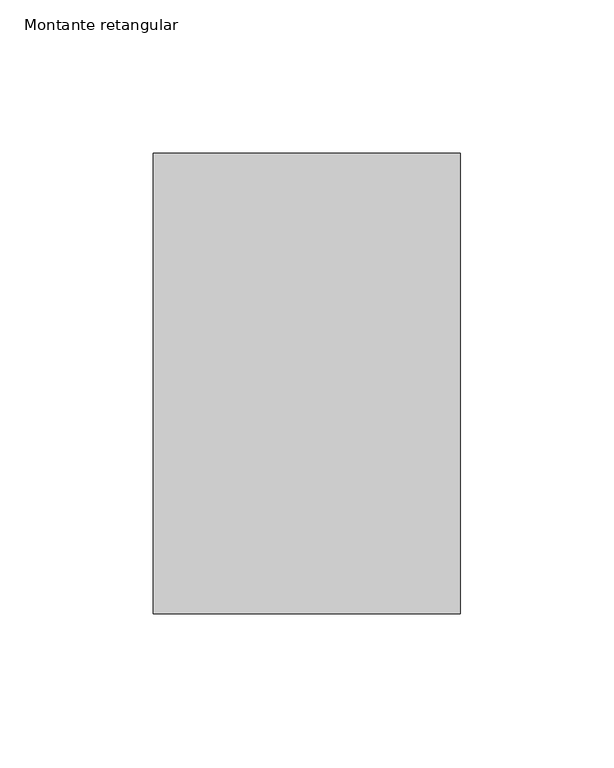
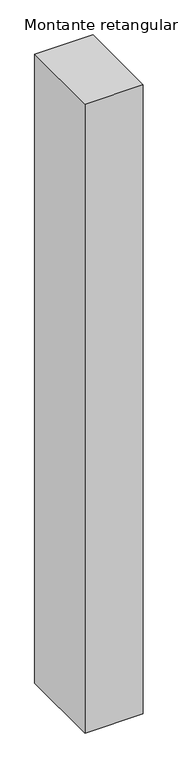
"""IFC4 building model written with IfcOpenShell, lengths in millimetres: member geometry, Montante retangular : CC_100 X 150  mm."""

import ifcopenshell
import ifcopenshell.guid

model = None  # the IFC model being written
_history = None  # IfcOwnerHistory: only IFC2X3 demands one
_inside = {}  # id of a spatial element -> (the spatial element, [elements in it])
_under = {}  # id of a project, library or spatial element -> (it, [spatial elements below it])
_declared = {}  # id of a project -> (the project, [libraries it declares])
_typed = {}  # id of a type object -> (the type object, [elements of that type])
_made_of = {}  # id of a material, layer set ... -> (it, [elements and type objects made of it])


def new_model(schema):
    """Start an empty IFC model of exactly this schema.

    Asked for "IFC4X3", IfcOpenShell would pick the latest addendum, in which some entities
    have other attributes; the version numbers below select the first issue.
    IFC2X3 requires an IfcOwnerHistory on every rooted entity: one is made here for all.
    """
    global model, _history
    if schema == "IFC4X3":
        model = ifcopenshell.file(schema_version=(4, 3, 0, 0))
    else:
        model = ifcopenshell.file(schema=schema)
    _inside.clear()
    _under.clear()
    _declared.clear()
    _typed.clear()
    _made_of.clear()
    _history = None
    if model.schema == "IFC2X3":
        org = make("IfcOrganization", Name="unknown")
        user = make(
            "IfcPersonAndOrganization",
            ThePerson=make("IfcPerson", FamilyName="unknown"),
            TheOrganization=org,
        )
        app = make(
            "IfcApplication",
            ApplicationDeveloper=org,
            Version="unknown",
            ApplicationFullName="unknown",
            ApplicationIdentifier="unknown",
        )
        _history = make(
            "IfcOwnerHistory",
            OwningUser=user,
            OwningApplication=app,
            ChangeAction="ADDED",
            CreationDate=0,
        )
    return model


def make(cls, **values):
    """One entity of the class cls with the attributes given. An attribute that is None is left unset."""
    return model.create_entity(
        cls, **{name: value for name, value in values.items() if value is not None}
    )


def rooted(cls, **values):
    """An entity with a GlobalId (a new one), such as an element, a storey or a relation."""
    return make(cls, GlobalId=ifcopenshell.guid.new(), OwnerHistory=_history, **values)


def si_unit(unit_type, name, prefix=None):
    """IfcSIUnit, for example si_unit("LENGTHUNIT", "METRE", prefix="MILLI")."""
    return make("IfcSIUnit", UnitType=unit_type, Prefix=prefix, Name=name)


def assignment(units):
    """IfcUnitAssignment: the units of a project."""
    return None if units is None else make("IfcUnitAssignment", Units=units)


def point(xyz):
    """IfcCartesianPoint."""
    return None if xyz is None else make("IfcCartesianPoint", Coordinates=xyz)


def direction(xyz):
    """IfcDirection."""
    return None if xyz is None else make("IfcDirection", DirectionRatios=xyz)


def frame(location, z_axis=None, x_axis=None):
    """IfcAxis2Placement3D, a coordinate frame: its origin and axes. An axis left out is left unset."""
    return make(
        "IfcAxis2Placement3D",
        Location=point(location),
        Axis=direction(z_axis),
        RefDirection=direction(x_axis),
    )


def origin():
    """The frame at (0, 0, 0) with its axes left unset."""
    return frame((0.0, 0.0, 0.0))


def place(relative_to, where):
    """IfcLocalPlacement: puts the frame where relative to a parent placement (None: the world)."""
    return make(
        "IfcLocalPlacement", PlacementRelTo=relative_to, RelativePlacement=where
    )


def context(
    kind, dimensions, precision=None, world=None, true_north=None, identifier=None
):
    """IfcGeometricRepresentationContext, for example the 3D "Model" context."""
    return make(
        "IfcGeometricRepresentationContext",
        ContextIdentifier=identifier,
        ContextType=kind,
        CoordinateSpaceDimension=dimensions,
        Precision=precision,
        WorldCoordinateSystem=world,
        TrueNorth=true_north,
    )


def project(units=None, contexts=None):
    """IfcProject with its units and contexts."""
    return rooted(
        "IfcProject",
        Name="project",
        RepresentationContexts=contexts,
        UnitsInContext=assignment(units),
    )


def spatial(cls, under=None, at=None, **own):
    """A site, building, storey or space (cls), placed at a placement, below another one or the project."""
    s = rooted(cls, ObjectPlacement=at, **own)
    if under is not None:
        _under.setdefault(under.id(), (under, []))[1].append(s)
    return s


def polyline(points):
    """IfcPolyline through the points."""
    return make("IfcPolyline", Points=[point(p) for p in points])


def outline(outer, holes=None, kind="AREA"):
    """IfcArbitraryClosedProfileDef: a profile drawn as a closed curve; with holes, ...WithVoids."""
    if holes is None:
        return make("IfcArbitraryClosedProfileDef", ProfileType=kind, OuterCurve=outer)
    return make(
        "IfcArbitraryProfileDefWithVoids",
        ProfileType=kind,
        OuterCurve=outer,
        InnerCurves=holes,
    )


def extrude(swept, where, along, depth):
    """IfcExtrudedAreaSolid: the profile swept, set in the frame where, extruded along a direction by depth."""
    return make(
        "IfcExtrudedAreaSolid",
        SweptArea=swept,
        Position=where,
        ExtrudedDirection=direction(along),
        Depth=depth,
    )


def shape(context_of_items, identifier, shape_type, items):
    """IfcShapeRepresentation: the items that make up one representation, for example the "Body"."""
    return make(
        "IfcShapeRepresentation",
        ContextOfItems=context_of_items,
        RepresentationIdentifier=identifier,
        RepresentationType=shape_type,
        Items=items,
    )


def source(mapping_origin, context_of_items, identifier, shape_type, items):
    """IfcRepresentationMap: a shape defined once, which mapped items show again and again."""
    return make(
        "IfcRepresentationMap",
        MappingOrigin=mapping_origin,
        MappedRepresentation=shape(context_of_items, identifier, shape_type, items),
    )


def transform(
    local_origin,
    x_axis=None,
    y_axis=None,
    z_axis=None,
    scale=None,
    scale2=None,
    scale3=None,
    uniform=True,
):
    """IfcCartesianTransformationOperator3D, or its non-uniform kind. x_axis, y_axis, z_axis: its Axis1, 2, 3."""
    if uniform:
        return make(
            "IfcCartesianTransformationOperator3D",
            Axis1=direction(x_axis),
            Axis2=direction(y_axis),
            LocalOrigin=point(local_origin),
            Scale=scale,
            Axis3=direction(z_axis),
        )
    return make(
        "IfcCartesianTransformationOperator3DnonUniform",
        Axis1=direction(x_axis),
        Axis2=direction(y_axis),
        LocalOrigin=point(local_origin),
        Scale=scale,
        Axis3=direction(z_axis),
        Scale2=scale2,
        Scale3=scale3,
    )


def mapped(mapping_source, mapping_target):
    """IfcMappedItem: shows the shape of a source again, moved by a transform."""
    return make(
        "IfcMappedItem", MappingSource=mapping_source, MappingTarget=mapping_target
    )


def made_of(thing, what):
    """Note that an element or type object is made of a material, layer set ...; save() writes the relation."""
    if what is not None:
        _made_of.setdefault(what.id(), (what, []))[1].append(thing)
    return thing


def element(
    cls,
    number,
    at=None,
    inside=None,
    cuts=None,
    type_object=None,
    material=None,
    context=None,
    identifier="Body",
    shape_type=None,
    held_by="IfcProductDefinitionShape",
    body=None,
    shapes=None,
    **own,
):
    """One element of the class cls, such as IfcWall. Its Tag is "e" and its number.

    at: its placement. inside: the storey or other place that contains it. cuts: it is an
    opening in that element (IfcRelVoidsElement). A single representation is given by context,
    identifier, shape_type and body (its items); several are given by shapes. held_by: the class
    of the entity that holds the representations. save() writes the other relations.
    """
    e = rooted(cls, Tag="e%d" % number, ObjectPlacement=at, **own)
    if body is not None:
        shapes = [shape(context, identifier, shape_type, body)]
    if shapes is not None:
        e.Representation = make(held_by, Representations=shapes)
    if inside is not None:
        _inside.setdefault(inside.id(), (inside, []))[1].append(e)
    if cuts is not None:
        rooted(
            "IfcRelVoidsElement", RelatingBuildingElement=cuts, RelatedOpeningElement=e
        )
    if type_object is not None:
        _typed.setdefault(type_object.id(), (type_object, []))[1].append(e)
    return made_of(e, material)


def aggregate(whole, parts):
    """IfcRelAggregates: a whole, such as a stair, and the parts it consists of."""
    return rooted("IfcRelAggregates", RelatingObject=whole, RelatedObjects=parts)


def save(model, path):
    """Write the relations noted so far, then the file.

    IfcRelAggregates (storeys below a building ...), IfcRelContainedInSpatialStructure (elements
    in a storey), IfcRelDefinesByType, IfcRelAssociatesMaterial and IfcRelDeclares: one each for
    every whole, place, type object, material and project.
    """
    for whole, parts in _under.values():
        aggregate(whole, parts)
    for where, things in _inside.values():
        rooted(
            "IfcRelContainedInSpatialStructure",
            RelatedElements=things,
            RelatingStructure=where,
        )
    for kind, things in _typed.values():
        rooted("IfcRelDefinesByType", RelatedObjects=things, RelatingType=kind)
    for what, things in _made_of.values():
        rooted("IfcRelAssociatesMaterial", RelatedObjects=things, RelatingMaterial=what)
    for by, libraries in _declared.values():
        rooted("IfcRelDeclares", RelatingContext=by, RelatedDefinitions=libraries)
    model.write(path)


def montante_retangular_d0ec09bd(model_context):
    return source(origin(), model_context, "Body", "SweptSolid", [
        extrude(outline(polyline([(50.0, 75.0), (50.0, -75.0), (-50.0, -75.0), (-50.0, 75.0), (50.0, 75.0)])), frame((0.0, 0.0, -1143.7500002), z_axis=(0.0, 0.0, 1.0), x_axis=(1.0, 0.0, 0.0)), (0.0, 0.0, 1.0), 1143.7500002),
    ])


if __name__ == "__main__":
    model = new_model("IFC4")
    model_context = context("Model", 3, world=origin())
    ifc_project = project(units=[si_unit("LENGTHUNIT", "METRE", prefix="MILLI")], contexts=[model_context])
    site = spatial("IfcSite", under=ifc_project)
    building = spatial("IfcBuilding", under=site)
    placement = place(None, origin())
    montante_retangular_shape = montante_retangular_d0ec09bd(model_context)
    element("IfcMember", 1, ObjectType="Montante retangular : CC_100 X 150  mm", at=placement, inside=building, context=model_context, shape_type="MappedRepresentation", body=[
        mapped(montante_retangular_shape, transform((0.0, 0.0, 0.0), x_axis=(1.0, 0.0, 0.0), y_axis=(0.0, 1.0, 0.0), z_axis=(0.0, 0.0, 1.0))),
    ])
    save(model, "model.ifc")

# Revit data of these elements
# Type "Montante retangular : CC_100 X 150  mm"
#   built-in parameter 1007304 = 0.492126 (stored number, unit not read)
#   built-in parameter 1007301 = 0.164042 (stored number, unit not read)
#   built-in parameter 1007300 = 0.164042 (stored number, unit not read)
# Element 1 (IfcMember, "Montante retangular : CC_100 X 150  mm")
#   Materials on its faces: ".ALUMÍNIO"
# Materials
#   ".ALUMÍNIO": class "CC_METAIS", colour RGB 244 244 244, transparency 0, Description = "Material alumínio", Cost = 0
